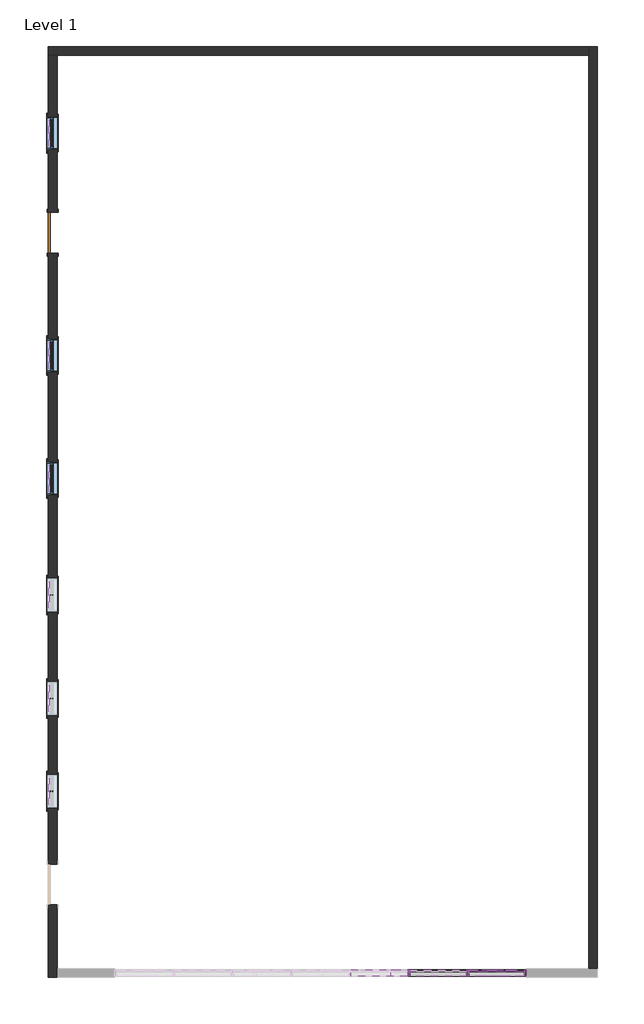
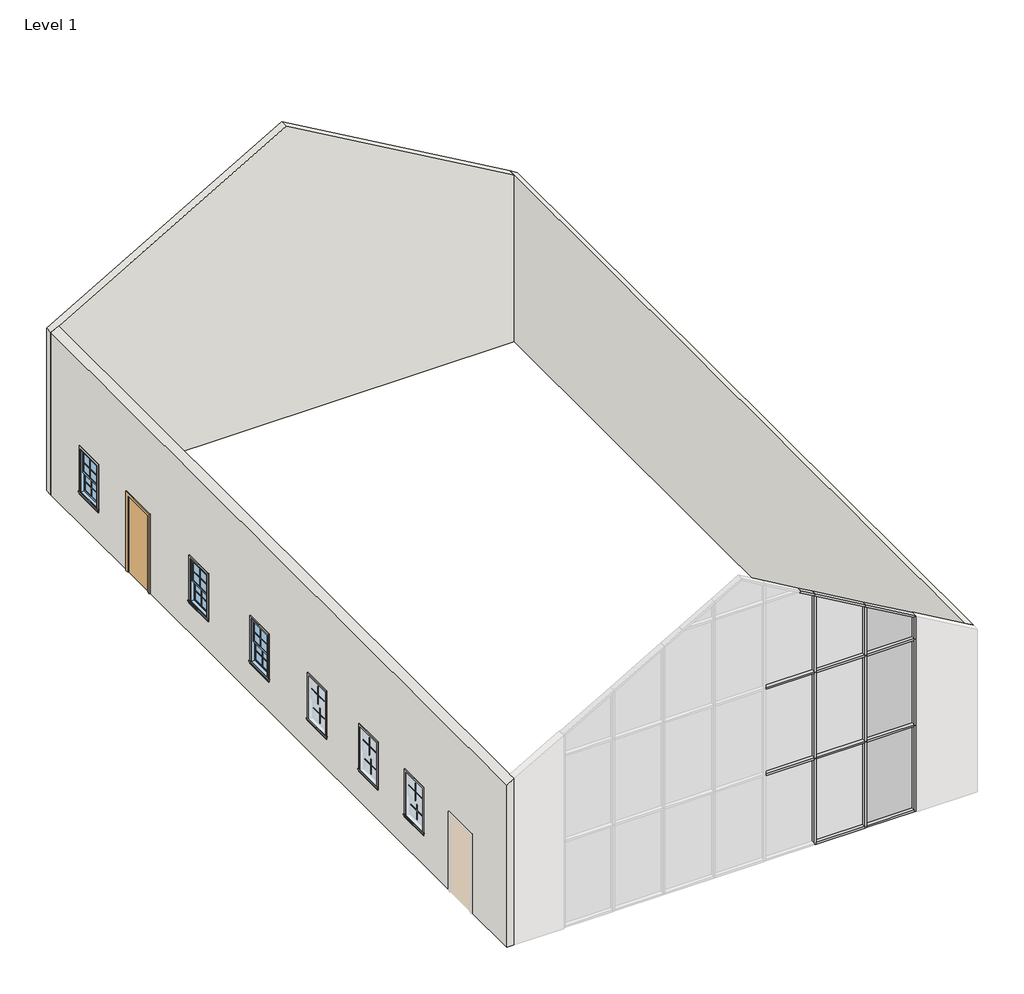
# One storey, part 2 of 2: 24 proxies, 20 members, 3 plates, 3 walls, 3 windows, 1 door.
"""IFC4 building model written with IfcOpenShell, lengths in millimetres."""

import ifcopenshell
import ifcopenshell.guid

model = None  # the IFC model being written
_history = None  # IfcOwnerHistory: only IFC2X3 demands one
_inside = {}  # id of a spatial element -> (the spatial element, [elements in it])
_under = {}  # id of a project, library or spatial element -> (it, [spatial elements below it])
_declared = {}  # id of a project -> (the project, [libraries it declares])
_typed = {}  # id of a type object -> (the type object, [elements of that type])
_made_of = {}  # id of a material, layer set ... -> (it, [elements and type objects made of it])


def new_model(schema):
    """Start an empty IFC model of exactly this schema.

    Asked for "IFC4X3", IfcOpenShell would pick the latest addendum, in which some entities
    have other attributes; the version numbers below select the first issue.
    IFC2X3 requires an IfcOwnerHistory on every rooted entity: one is made here for all.
    """
    global model, _history
    if schema == "IFC4X3":
        model = ifcopenshell.file(schema_version=(4, 3, 0, 0))
    else:
        model = ifcopenshell.file(schema=schema)
    _inside.clear()
    _under.clear()
    _declared.clear()
    _typed.clear()
    _made_of.clear()
    _history = None
    if model.schema == "IFC2X3":
        org = make("IfcOrganization", Name="unknown")
        user = make(
            "IfcPersonAndOrganization",
            ThePerson=make("IfcPerson", FamilyName="unknown"),
            TheOrganization=org,
        )
        app = make(
            "IfcApplication",
            ApplicationDeveloper=org,
            Version="unknown",
            ApplicationFullName="unknown",
            ApplicationIdentifier="unknown",
        )
        _history = make(
            "IfcOwnerHistory",
            OwningUser=user,
            OwningApplication=app,
            ChangeAction="ADDED",
            CreationDate=0,
        )
    return model


def make(cls, **values):
    """One entity of the class cls with the attributes given. An attribute that is None is left unset."""
    return model.create_entity(
        cls, **{name: value for name, value in values.items() if value is not None}
    )


def rooted(cls, **values):
    """An entity with a GlobalId (a new one), such as an element, a storey or a relation."""
    return make(cls, GlobalId=ifcopenshell.guid.new(), OwnerHistory=_history, **values)


def si_unit(unit_type, name, prefix=None):
    """IfcSIUnit, for example si_unit("LENGTHUNIT", "METRE", prefix="MILLI")."""
    return make("IfcSIUnit", UnitType=unit_type, Prefix=prefix, Name=name)


def assignment(units):
    """IfcUnitAssignment: the units of a project."""
    return None if units is None else make("IfcUnitAssignment", Units=units)


def point(xyz):
    """IfcCartesianPoint."""
    return None if xyz is None else make("IfcCartesianPoint", Coordinates=xyz)


def direction(xyz):
    """IfcDirection."""
    return None if xyz is None else make("IfcDirection", DirectionRatios=xyz)


def frame(location, z_axis=None, x_axis=None):
    """IfcAxis2Placement3D, a coordinate frame: its origin and axes. An axis left out is left unset."""
    return make(
        "IfcAxis2Placement3D",
        Location=point(location),
        Axis=direction(z_axis),
        RefDirection=direction(x_axis),
    )


def origin():
    """The frame at (0, 0, 0) with its axes left unset."""
    return frame((0.0, 0.0, 0.0))


def origin_with_axes():
    """The frame at (0, 0, 0) with the z axis (0, 0, 1) and the x axis (1, 0, 0) written out."""
    return frame((0.0, 0.0, 0.0), z_axis=(0.0, 0.0, 1.0), x_axis=(1.0, 0.0, 0.0))


def place(relative_to, where):
    """IfcLocalPlacement: puts the frame where relative to a parent placement (None: the world)."""
    return make(
        "IfcLocalPlacement", PlacementRelTo=relative_to, RelativePlacement=where
    )


def context(
    kind, dimensions, precision=None, world=None, true_north=None, identifier=None
):
    """IfcGeometricRepresentationContext, for example the 3D "Model" context."""
    return make(
        "IfcGeometricRepresentationContext",
        ContextIdentifier=identifier,
        ContextType=kind,
        CoordinateSpaceDimension=dimensions,
        Precision=precision,
        WorldCoordinateSystem=world,
        TrueNorth=true_north,
    )


def project(units=None, contexts=None):
    """IfcProject with its units and contexts."""
    return rooted(
        "IfcProject",
        Name="project",
        RepresentationContexts=contexts,
        UnitsInContext=assignment(units),
    )


def spatial(cls, under=None, at=None, **own):
    """A site, building, storey or space (cls), placed at a placement, below another one or the project."""
    s = rooted(cls, ObjectPlacement=at, **own)
    if under is not None:
        _under.setdefault(under.id(), (under, []))[1].append(s)
    return s


def polyline(points):
    """IfcPolyline through the points."""
    return make("IfcPolyline", Points=[point(p) for p in points])


def outline(outer, holes=None, kind="AREA"):
    """IfcArbitraryClosedProfileDef: a profile drawn as a closed curve; with holes, ...WithVoids."""
    if holes is None:
        return make("IfcArbitraryClosedProfileDef", ProfileType=kind, OuterCurve=outer)
    return make(
        "IfcArbitraryProfileDefWithVoids",
        ProfileType=kind,
        OuterCurve=outer,
        InnerCurves=holes,
    )


def extrude(swept, where, along, depth):
    """IfcExtrudedAreaSolid: the profile swept, set in the frame where, extruded along a direction by depth."""
    return make(
        "IfcExtrudedAreaSolid",
        SweptArea=swept,
        Position=where,
        ExtrudedDirection=direction(along),
        Depth=depth,
    )


def faces_of(points, faces, orient=None, outer=None):
    """IfcFace entities. A face is a list of loops; a loop is a list of indices into points, from 0.

    orient and outer hold one flag for each loop. By default every Orientation is true, the
    first loop of a face is its IfcFaceOuterBound and the others are IfcFaceBound.
    """
    made = []
    for i, loops in enumerate(faces):
        bounds = []
        for j, loop in enumerate(loops):
            is_outer = j == 0 if outer is None else outer[i][j]
            bounds.append(
                make(
                    "IfcFaceOuterBound" if is_outer else "IfcFaceBound",
                    Bound=make("IfcPolyLoop", Polygon=[points[k] for k in loop]),
                    Orientation=True if orient is None else orient[i][j],
                )
            )
        made.append(make("IfcFace", Bounds=bounds))
    return made


def faceted_brep(points, faces, orient=None, outer=None, voids=None):
    """IfcFacetedBrep: a solid bounded by flat faces; with voids (closed shells), ...WithVoids."""
    shared = [point(p) for p in points]
    hull = make("IfcClosedShell", CfsFaces=faces_of(shared, faces, orient, outer))
    if voids is None:
        return make("IfcFacetedBrep", Outer=hull)
    return make(
        "IfcFacetedBrepWithVoids",
        Outer=hull,
        Voids=[
            make(cls, CfsFaces=faces_of(shared, fs, o, b)) for cls, fs, o, b in voids
        ],
    )


def shape(context_of_items, identifier, shape_type, items):
    """IfcShapeRepresentation: the items that make up one representation, for example the "Body"."""
    return make(
        "IfcShapeRepresentation",
        ContextOfItems=context_of_items,
        RepresentationIdentifier=identifier,
        RepresentationType=shape_type,
        Items=items,
    )


def source(mapping_origin, context_of_items, identifier, shape_type, items):
    """IfcRepresentationMap: a shape defined once, which mapped items show again and again."""
    return make(
        "IfcRepresentationMap",
        MappingOrigin=mapping_origin,
        MappedRepresentation=shape(context_of_items, identifier, shape_type, items),
    )


def transform(
    local_origin,
    x_axis=None,
    y_axis=None,
    z_axis=None,
    scale=None,
    scale2=None,
    scale3=None,
    uniform=True,
):
    """IfcCartesianTransformationOperator3D, or its non-uniform kind. x_axis, y_axis, z_axis: its Axis1, 2, 3."""
    if uniform:
        return make(
            "IfcCartesianTransformationOperator3D",
            Axis1=direction(x_axis),
            Axis2=direction(y_axis),
            LocalOrigin=point(local_origin),
            Scale=scale,
            Axis3=direction(z_axis),
        )
    return make(
        "IfcCartesianTransformationOperator3DnonUniform",
        Axis1=direction(x_axis),
        Axis2=direction(y_axis),
        LocalOrigin=point(local_origin),
        Scale=scale,
        Axis3=direction(z_axis),
        Scale2=scale2,
        Scale3=scale3,
    )


def mapped(mapping_source, mapping_target):
    """IfcMappedItem: shows the shape of a source again, moved by a transform."""
    return make(
        "IfcMappedItem", MappingSource=mapping_source, MappingTarget=mapping_target
    )


def made_of(thing, what):
    """Note that an element or type object is made of a material, layer set ...; save() writes the relation."""
    if what is not None:
        _made_of.setdefault(what.id(), (what, []))[1].append(thing)
    return thing


def element(
    cls,
    number,
    at=None,
    inside=None,
    cuts=None,
    type_object=None,
    material=None,
    context=None,
    identifier="Body",
    shape_type=None,
    held_by="IfcProductDefinitionShape",
    body=None,
    shapes=None,
    **own,
):
    """One element of the class cls, such as IfcWall. Its Tag is "e" and its number.

    at: its placement. inside: the storey or other place that contains it. cuts: it is an
    opening in that element (IfcRelVoidsElement). A single representation is given by context,
    identifier, shape_type and body (its items); several are given by shapes. held_by: the class
    of the entity that holds the representations. save() writes the other relations.
    """
    e = rooted(cls, Tag="e%d" % number, ObjectPlacement=at, **own)
    if body is not None:
        shapes = [shape(context, identifier, shape_type, body)]
    if shapes is not None:
        e.Representation = make(held_by, Representations=shapes)
    if inside is not None:
        _inside.setdefault(inside.id(), (inside, []))[1].append(e)
    if cuts is not None:
        rooted(
            "IfcRelVoidsElement", RelatingBuildingElement=cuts, RelatedOpeningElement=e
        )
    if type_object is not None:
        _typed.setdefault(type_object.id(), (type_object, []))[1].append(e)
    return made_of(e, material)


def aggregate(whole, parts):
    """IfcRelAggregates: a whole, such as a stair, and the parts it consists of."""
    return rooted("IfcRelAggregates", RelatingObject=whole, RelatedObjects=parts)


def save(model, path):
    """Write the relations noted so far, then the file.

    IfcRelAggregates (storeys below a building ...), IfcRelContainedInSpatialStructure (elements
    in a storey), IfcRelDefinesByType, IfcRelAssociatesMaterial and IfcRelDeclares: one each for
    every whole, place, type object, material and project.
    """
    for whole, parts in _under.values():
        aggregate(whole, parts)
    for where, things in _inside.values():
        rooted(
            "IfcRelContainedInSpatialStructure",
            RelatedElements=things,
            RelatingStructure=where,
        )
    for kind, things in _typed.values():
        rooted("IfcRelDefinesByType", RelatedObjects=things, RelatingType=kind)
    for what, things in _made_of.values():
        rooted("IfcRelAssociatesMaterial", RelatedObjects=things, RelatingMaterial=what)
    for by, libraries in _declared.values():
        rooted("IfcRelDeclares", RelatingContext=by, RelatedDefinitions=libraries)
    model.write(path)


def m_muntin_pattern_2x2_m_muntin_pattern_2x2_aaec3afb(model_context):
    return source(origin(), model_context, "Body", "SweptSolid", [
        extrude(outline(polyline([(257.1375, -6.35), (257.1375, -298.8), (244.4375, -298.8), (244.4375, -6.35), (0.0, -6.35), (0.0, 6.35), (244.4375, 6.35), (244.4375, 298.8), (257.1375, 298.8), (257.1375, 6.35), (501.575, 6.35), (501.575, -6.35), (257.1375, -6.35)])), frame((0.0, 9.525, 0.0), z_axis=(0.0, 1.0, 0.0), x_axis=(0.0, 0.0, 1.0)), (0.0, 0.0, 1.0), 12.7),
        extrude(outline(polyline([(257.1375, -6.35), (257.1375, -298.8), (244.4375, -298.8), (244.4375, -6.35), (0.0, -6.35), (0.0, 6.35), (244.4375, 6.35), (244.4375, 298.8), (257.1375, 298.8), (257.1375, 6.35), (501.575, 6.35), (501.575, -6.35), (257.1375, -6.35)])), frame((0.0, -22.225, 0.0), z_axis=(0.0, 1.0, 0.0), x_axis=(0.0, 0.0, 1.0)), (0.0, 0.0, 1.0), 12.7),
    ])


def m_trim_window_exterior_flat_with_sill_e7ff6350(model_context):
    return source(origin(), model_context, "Body", "SweptSolid", [
        extrude(outline(polyline([(435.0, -1220.4323709), (435.0, -1280.4323709), (-435.0, -1280.4323709), (-435.0, -1220.4323709), (435.0, -1220.4323709)])), origin_with_axes(), (0.0, 0.0, 1.0), 19.05),
        extrude(outline(polyline([(-1230.0, 38.1), (-1202.4580645, 38.1), (-1200.0, 19.05), (-1200.0, 0.0), (-1220.4323709, 0.0), (-1220.4323709, 19.05), (-1230.0, 19.05), (-1230.0, 38.1)])), frame((-447.7, 0.0, 0.0), z_axis=(1.0, 0.0, 0.0), x_axis=(0.0, 1.0, 0.0)), (0.0, 0.0, 1.0), 895.4),
        extrude(outline(polyline([(-435.0, 60.0), (435.0, 60.0), (435.0, -1200.0), (375.0, -1200.0), (375.0, 0.0), (-375.0, 0.0), (-375.0, -1200.0), (-435.0, -1200.0), (-435.0, 60.0)])), origin_with_axes(), (0.0, 0.0, 1.0), 19.05),
    ])


def m_trim_window_interior_flat_picture_frame_31bd2320(model_context):
    return source(origin(), model_context, "Body", "SweptSolid", [
        extrude(outline(polyline([(422.3, 47.3), (422.3, -1247.3), (-422.3, -1247.3), (-422.3, 47.3), (422.3, 47.3)]), holes=[polyline([(362.3, -12.7), (-362.3, -12.7), (-362.3, -1187.3), (362.3, -1187.3), (362.3, -12.7)])]), origin_with_axes(), (0.0, 0.0, 1.0), 30.0),
    ])


def m_single_flush_0915_x_2134mm_6a9e8738(model_context):
    return source(origin(), model_context, "Body", "SweptSolid", [
        extrude(outline(polyline([(2210.0, -533.5), (0.0, -533.5), (0.0, -457.5), (2134.0, -457.5), (2134.0, 457.5), (0.0, 457.5), (0.0, 533.5), (2210.0, 533.5), (2210.0, -533.5)])), frame((0.0, 100.0, 0.0), z_axis=(0.0, 1.0, 0.0), x_axis=(0.0, 0.0, 1.0)), (0.0, 0.0, 1.0), 25.0),
        extrude(outline(polyline([(2210.0, 533.5), (2210.0, -533.5), (0.0, -533.5), (0.0, -457.5), (2134.0, -457.5), (2134.0, 457.5), (0.0, 457.5), (0.0, 533.5), (2210.0, 533.5)])), frame((0.0, -125.0, 0.0), z_axis=(0.0, 1.0, 0.0), x_axis=(0.0, 0.0, 1.0)), (0.0, 0.0, 1.0), 25.0),
        extrude(outline(polyline([(457.5, 49.0), (-457.5, 49.0), (-457.5, 100.0), (457.5, 100.0), (457.5, 49.0)])), origin_with_axes(), (0.0, 0.0, 1.0), 2134.0),
    ])


def rectangular_mullion_50mm_x_150mm_302a0cfa(model_context):
    return source(origin(), model_context, "Body", "SweptSolid", [
        extrude(outline(polyline([(0.0, 75.0), (0.0, -75.0), (-50.0, -75.0), (-50.0, 75.0), (0.0, 75.0)])), frame((0.0, 0.0, -1253.5714288), z_axis=(0.0, 0.0, 1.0), x_axis=(1.0, 0.0, 0.0)), (0.0, 0.0, 1.0), 1253.5714288),
    ])


def rectangular_mullion_50mm_x_150mm_11a5ee59(model_context):
    return source(origin(), model_context, "Body", "SweptSolid", [
        extrude(outline(polyline([(0.0, 75.0), (0.0, -75.0), (-50.0, -75.0), (-50.0, 75.0), (0.0, 75.0)])), frame((0.0, 0.0, -1278.5714285), z_axis=(0.0, 0.0, 1.0), x_axis=(1.0, 0.0, 0.0)), (0.0, 0.0, 1.0), 1278.5714285),
    ])


def rectangular_mullion_50mm_x_150mm_46426fc7(model_context):
    return source(origin(), model_context, "Body", "SweptSolid", [
        extrude(outline(polyline([(25.0, 75.0), (25.0, -75.0), (-25.0, -75.0), (-25.0, 75.0), (25.0, 75.0)])), frame((0.0, 0.0, -1253.5714288), z_axis=(0.0, 0.0, 1.0), x_axis=(1.0, 0.0, 0.0)), (0.0, 0.0, 1.0), 1253.5714288),
    ])


def rectangular_mullion_50mm_x_150mm_f38f42f6(model_context):
    return source(origin(), model_context, "Body", "SweptSolid", [
        extrude(outline(polyline([(25.0, 75.0), (25.0, -75.0), (-25.0, -75.0), (-25.0, 75.0), (25.0, 75.0)])), frame((0.0, 0.0, -1278.5714285), z_axis=(0.0, 0.0, 1.0), x_axis=(1.0, 0.0, 0.0)), (0.0, 0.0, 1.0), 1278.5714285),
    ])


def rectangular_mullion_50mm_x_150mm_6225e4e3(model_context):
    return source(origin(), model_context, "Body", "SweptSolid", [
        extrude(outline(polyline([(25.0, 75.0), (25.0, -75.0), (-25.0, -75.0), (-25.0, 75.0), (25.0, 75.0)])), frame((0.0, 0.0, -2400.0), z_axis=(0.0, 0.0, 1.0), x_axis=(1.0, 0.0, 0.0)), (0.0, 0.0, 1.0), 2400.0),
    ])


def rectangular_mullion_50mm_x_150mm_662c37b1(model_context):
    return source(origin(), model_context, "Body", "SweptSolid", [
        extrude(outline(polyline([(0.0, 75.0), (0.0, -75.0), (-50.0, -75.0), (-50.0, 75.0), (0.0, 75.0)])), frame((0.0, 0.0, -2400.0), z_axis=(0.0, 0.0, 1.0), x_axis=(1.0, 0.0, 0.0)), (0.0, 0.0, 1.0), 2400.0),
    ])


def rectangular_mullion_50mm_x_150mm_c4d7f9a4(model_context):
    return source(origin(), model_context, "Body", "SweptSolid", [
        extrude(outline(polyline([(0.0, 25.0), (0.0, -25.0), (-2134.1765467, -25.0), (-2105.3090332, 25.0), (0.0, 25.0)])), frame((0.0, -75.0, 0.0), z_axis=(0.0, 1.0, 0.0), x_axis=(0.0, 0.0, 1.0)), (0.0, 0.0, 1.0), 150.0),
    ])


def rectangular_mullion_50mm_x_150mm_5374cabd(model_context):
    return source(origin(), model_context, "Body", "SweptSolid", [
        extrude(outline(polyline([(0.0, 25.0), (0.0, -25.0), (-1367.1254748, -25.0), (-1338.2579614, 25.0), (0.0, 25.0)])), frame((0.0, -75.0, 0.0), z_axis=(0.0, 1.0, 0.0), x_axis=(0.0, 0.0, 1.0)), (0.0, 0.0, 1.0), 150.0),
    ])


def rectangular_mullion_50mm_x_150mm_03c50f69(model_context):
    return source(origin(), model_context, "Body", "SweptSolid", [
        extrude(outline(polyline([(0.0, 0.0), (-28.8675135, -50.0), (-1534.1021441, -50.0), (-1534.1021441, 0.0), (0.0, 0.0)])), frame((0.0, -75.0, 0.0), z_axis=(0.0, 1.0, 0.0), x_axis=(0.0, 0.0, 1.0)), (0.0, 0.0, 1.0), 150.0),
    ])


def rectangular_mullion_50mm_x_150mm_ffb0b627(model_context):
    return source(origin(), model_context, "Body", "SweptSolid", [
        extrude(outline(polyline([(0.0, 75.0), (0.0, -75.0), (-50.0, -75.0), (-50.0, 75.0), (0.0, 75.0)])), frame((0.0, 0.0, -445.0443662), z_axis=(0.0, 0.0, 1.0), x_axis=(1.0, 0.0, 0.0)), (0.0, 0.0, 1.0), 445.0443662),
    ])


def rectangular_mullion_50mm_x_150mm_95afd124(model_context):
    return source(origin(), model_context, "Body", "SweptSolid", [
        extrude(outline(polyline([(0.0, 75.0), (0.0, -75.0), (-50.0, -75.0), (-50.0, 75.0), (0.0, 75.0)])), frame((0.0, 0.0, -1534.1021437), z_axis=(0.0, 0.0, 1.0), x_axis=(1.0, 0.0, 0.0)), (0.0, 0.0, 1.0), 1534.1021437),
    ])


def rectangular_mullion_50mm_x_150mm_b704ab83(model_context):
    return source(origin(), model_context, "Body", "SweptSolid", [
        extrude(outline(polyline([(0.0, 0.0), (0.0, -50.0), (-614.5081595, -50.0), (-643.375673, 0.0), (0.0, 0.0)])), frame((0.0, -75.0, 0.0), z_axis=(0.0, 1.0, 0.0), x_axis=(0.0, 0.0, 1.0)), (0.0, 0.0, 1.0), 150.0),
    ])


def system_panel_glazed_b60b372a(model_context):
    return source(origin(), model_context, "Body", "SweptSolid", [
        extrude(outline(polyline([(626.7857144, 24.5), (-626.7857144, 24.5), (-626.7857144, 49.5), (626.7857144, 49.5), (626.7857144, 24.5)])), origin_with_axes(), (0.0, 0.0, 1.0), 2325.0),
    ])


def system_panel_glazed_eec4e8b3(model_context):
    return source(origin(), model_context, "Body", "SweptSolid", [
        extrude(outline(polyline([(626.7857144, 24.5), (-626.7857144, 24.5), (-626.7857144, 49.5), (626.7857144, 49.5), (626.7857144, 24.5)])), origin_with_axes(), (0.0, 0.0, 1.0), 2350.0),
    ])


def system_panel_glazed_62c7097b(model_context):
    return source(origin(), model_context, "Body", "SweptSolid", [
        extrude(outline(polyline([(0.0, -626.7857144), (0.0, 626.7857144), (589.5081595, 626.7857144), (1313.2579614, -626.7857144), (0.0, -626.7857144)])), frame((0.0, 24.5, 0.0), z_axis=(0.0, 1.0, 0.0), x_axis=(0.0, 0.0, 1.0)), (0.0, 0.0, 1.0), 25.0),
    ])


def m_window_double_hung_750_x_1200mm_41070976(model_context):
    return source(origin(), model_context, "Body", "SweptSolid", [
        extrude(outline(polyline([(298.8, 30.15), (298.8, 23.8), (-298.8, 23.8), (-298.8, 30.15), (298.8, 30.15)])), frame((0.0, 0.0, 990.6), z_axis=(0.0, 0.0, 1.0), x_axis=(1.0, 0.0, 0.0)), (0.0, 0.0, 1.0), 501.575),
        extrude(outline(polyline([(-298.8, 17.45), (298.8, 17.45), (298.8, 11.1), (-298.8, 11.1), (-298.8, 17.45)])), frame((0.0, 0.0, 990.6), z_axis=(0.0, 0.0, 1.0), x_axis=(1.0, 0.0, 0.0)), (0.0, 0.0, 1.0), 501.575),
        extrude(outline(polyline([(298.8, 74.6), (298.8, 68.25), (-298.8, 68.25), (-298.8, 74.6), (298.8, 74.6)])), frame((0.0, 0.0, 1536.625), z_axis=(0.0, 0.0, 1.0), x_axis=(1.0, 0.0, 0.0)), (0.0, 0.0, 1.0), 501.575),
        extrude(outline(polyline([(-298.8, 61.9), (298.8, 61.9), (298.8, 55.55), (-298.8, 55.55), (-298.8, 61.9)])), frame((0.0, 0.0, 1536.625), z_axis=(0.0, 0.0, 1.0), x_axis=(1.0, 0.0, 0.0)), (0.0, 0.0, 1.0), 501.575),
        extrude(outline(polyline([(1536.625, -343.25), (946.15, -343.25), (946.15, 343.25), (1536.625, 343.25), (1536.625, -343.25)]), holes=[polyline([(1492.175, 298.8), (990.6, 298.8), (990.6, -298.8), (1492.175, -298.8), (1492.175, 298.8)])]), frame((0.0, -1.6, 0.0), z_axis=(0.0, 1.0, 0.0), x_axis=(0.0, 0.0, 1.0)), (0.0, 0.0, 1.0), 44.45),
        extrude(outline(polyline([(2082.65, -343.25), (1492.175, -343.25), (1492.175, 343.25), (2082.65, 343.25), (2082.65, -343.25)]), holes=[polyline([(2038.2, 298.8), (1536.625, 298.8), (1536.625, -298.8), (2038.2, -298.8), (2038.2, 298.8)])]), frame((0.0, 42.85, 0.0), z_axis=(0.0, 1.0, 0.0), x_axis=(0.0, 0.0, 1.0)), (0.0, 0.0, 1.0), 44.45),
        extrude(outline(polyline([(2114.4, -375.0), (914.4, -375.0), (914.4, 375.0), (2114.4, 375.0), (2114.4, -375.0)]), holes=[polyline([(2082.65, 343.25), (946.15, 343.25), (946.15, -343.25), (2082.65, -343.25), (2082.65, 343.25)])]), frame((0.0, -14.3, 0.0), z_axis=(0.0, 1.0, 0.0), x_axis=(0.0, 0.0, 1.0)), (0.0, 0.0, 1.0), 133.35),
        extrude(outline(polyline([(2114.4, 375.0), (2114.4, -375.0), (914.4, -375.0), (914.4, 375.0), (2114.4, 375.0)]), holes=[polyline([(2095.35, 355.95), (933.45, 355.95), (933.45, -355.95), (2095.35, -355.95), (2095.35, 355.95)])]), frame((0.0, -100.0, 0.0), z_axis=(0.0, 1.0, 0.0), x_axis=(0.0, 0.0, 1.0)), (0.0, 0.0, 1.0), 85.7),
    ])


model = new_model("IFC4")

# Units and contexts
model_context = context("Model", 3, world=origin())
ifc_project = project(units=[si_unit("LENGTHUNIT", "METRE", prefix="MILLI")], contexts=[model_context])

# Site, building, storey
site = spatial("IfcSite", under=ifc_project)
building = spatial("IfcBuilding", under=site)
storey = spatial("IfcBuildingStorey", under=building, Name="Level 1", Elevation=0.0)

# Proxies
placement = place(None, origin())
m_muntin_pattern_2x2_m_muntin_pattern_2x2_shape = m_muntin_pattern_2x2_m_muntin_pattern_2x2_aaec3afb(model_context)
element("IfcBuildingElementProxy", 1, Name="M_Muntin Pattern_2x2 : M_Muntin Pattern_2x2", ObjectType="M_Muntin Pattern_2x2 : M_Muntin Pattern_2x2", at=placement, inside=storey, context=model_context, shape_type="MappedRepresentation", body=[
    mapped(m_muntin_pattern_2x2_m_muntin_pattern_2x2_shape, transform((-7032.909392, -4566.9793434, 1536.625), x_axis=(0.0, 1.0, 0.0), y_axis=(-1.0, 0.0, 0.0), z_axis=(0.0, 0.0, 1.0))),
])
element("IfcBuildingElementProxy", 2, Name="M_Muntin Pattern_2x2 : M_Muntin Pattern_2x2", ObjectType="M_Muntin Pattern_2x2 : M_Muntin Pattern_2x2", at=placement, inside=storey, context=model_context, shape_type="MappedRepresentation", body=[
    mapped(m_muntin_pattern_2x2_m_muntin_pattern_2x2_shape, transform((-6988.459392, -4566.9793434, 990.6), x_axis=(0.0, 1.0, 0.0), y_axis=(-1.0, 0.0, 0.0), z_axis=(0.0, 0.0, 1.0))),
])
element("IfcBuildingElementProxy", 3, Name="M_Muntin Pattern_2x2 : M_Muntin Pattern_2x2", ObjectType="M_Muntin Pattern_2x2 : M_Muntin Pattern_2x2", at=placement, inside=storey, context=model_context, shape_type="MappedRepresentation", body=[
    mapped(m_muntin_pattern_2x2_m_muntin_pattern_2x2_shape, transform((-7032.909392, -2474.0000934, 1536.625), x_axis=(0.0, 1.0, 0.0), y_axis=(-1.0, 0.0, 0.0), z_axis=(0.0, 0.0, 1.0))),
])
element("IfcBuildingElementProxy", 4, Name="M_Muntin Pattern_2x2 : M_Muntin Pattern_2x2", ObjectType="M_Muntin Pattern_2x2 : M_Muntin Pattern_2x2", at=placement, inside=storey, context=model_context, shape_type="MappedRepresentation", body=[
    mapped(m_muntin_pattern_2x2_m_muntin_pattern_2x2_shape, transform((-6988.459392, -2474.0000934, 990.6), x_axis=(0.0, 1.0, 0.0), y_axis=(-1.0, 0.0, 0.0), z_axis=(0.0, 0.0, 1.0))),
])
element("IfcBuildingElementProxy", 5, Name="M_Muntin Pattern_2x2 : M_Muntin Pattern_2x2", ObjectType="M_Muntin Pattern_2x2 : M_Muntin Pattern_2x2", at=placement, inside=storey, context=model_context, shape_type="MappedRepresentation", body=[
    mapped(m_muntin_pattern_2x2_m_muntin_pattern_2x2_shape, transform((-7032.909392, -137.6511631, 1536.625), x_axis=(0.0, 1.0, 0.0), y_axis=(-1.0, 0.0, 0.0), z_axis=(0.0, 0.0, 1.0))),
])
element("IfcBuildingElementProxy", 6, Name="M_Muntin Pattern_2x2 : M_Muntin Pattern_2x2", ObjectType="M_Muntin Pattern_2x2 : M_Muntin Pattern_2x2", at=placement, inside=storey, context=model_context, shape_type="MappedRepresentation", body=[
    mapped(m_muntin_pattern_2x2_m_muntin_pattern_2x2_shape, transform((-6988.459392, -137.6511631, 990.6), x_axis=(0.0, 1.0, 0.0), y_axis=(-1.0, 0.0, 0.0), z_axis=(0.0, 0.0, 1.0))),
])
element("IfcBuildingElementProxy", 7, Name="M_Muntin Pattern_2x2 : M_Muntin Pattern_2x2", ObjectType="M_Muntin Pattern_2x2 : M_Muntin Pattern_2x2", at=placement, inside=storey, context=model_context, shape_type="MappedRepresentation", body=[
    mapped(m_muntin_pattern_2x2_m_muntin_pattern_2x2_shape, transform((-7032.909392, 2490.7413834, 1536.625), x_axis=(0.0, 1.0, 0.0), y_axis=(-1.0, 0.0, 0.0), z_axis=(0.0, 0.0, 1.0))),
])
element("IfcBuildingElementProxy", 8, Name="M_Muntin Pattern_2x2 : M_Muntin Pattern_2x2", ObjectType="M_Muntin Pattern_2x2 : M_Muntin Pattern_2x2", at=placement, inside=storey, context=model_context, shape_type="MappedRepresentation", body=[
    mapped(m_muntin_pattern_2x2_m_muntin_pattern_2x2_shape, transform((-6988.459392, 2490.7413834, 990.6), x_axis=(0.0, 1.0, 0.0), y_axis=(-1.0, 0.0, 0.0), z_axis=(0.0, 0.0, 1.0))),
])
element("IfcBuildingElementProxy", 9, Name="M_Muntin Pattern_2x2 : M_Muntin Pattern_2x2", ObjectType="M_Muntin Pattern_2x2 : M_Muntin Pattern_2x2", at=placement, inside=storey, context=model_context, shape_type="MappedRepresentation", body=[
    mapped(m_muntin_pattern_2x2_m_muntin_pattern_2x2_shape, transform((-7032.909392, 5265.1557382, 1536.625), x_axis=(0.0, 1.0, 0.0), y_axis=(-1.0, 0.0, 0.0), z_axis=(0.0, 0.0, 1.0))),
])
element("IfcBuildingElementProxy", 10, Name="M_Muntin Pattern_2x2 : M_Muntin Pattern_2x2", ObjectType="M_Muntin Pattern_2x2 : M_Muntin Pattern_2x2", at=placement, inside=storey, context=model_context, shape_type="MappedRepresentation", body=[
    mapped(m_muntin_pattern_2x2_m_muntin_pattern_2x2_shape, transform((-6988.459392, 5265.1557382, 990.6), x_axis=(0.0, 1.0, 0.0), y_axis=(-1.0, 0.0, 0.0), z_axis=(0.0, 0.0, 1.0))),
])
element("IfcBuildingElementProxy", 11, Name="M_Muntin Pattern_2x2 : M_Muntin Pattern_2x2", ObjectType="M_Muntin Pattern_2x2 : M_Muntin Pattern_2x2", at=placement, inside=storey, context=model_context, shape_type="MappedRepresentation", body=[
    mapped(m_muntin_pattern_2x2_m_muntin_pattern_2x2_shape, transform((-7032.909392, 10278.571151, 1536.625), x_axis=(0.0, 1.0, 0.0), y_axis=(-1.0, 0.0, 0.0), z_axis=(0.0, 0.0, 1.0))),
])
element("IfcBuildingElementProxy", 12, Name="M_Muntin Pattern_2x2 : M_Muntin Pattern_2x2", ObjectType="M_Muntin Pattern_2x2 : M_Muntin Pattern_2x2", at=placement, inside=storey, context=model_context, shape_type="MappedRepresentation", body=[
    mapped(m_muntin_pattern_2x2_m_muntin_pattern_2x2_shape, transform((-6988.459392, 10278.571151, 990.6), x_axis=(0.0, 1.0, 0.0), y_axis=(-1.0, 0.0, 0.0), z_axis=(0.0, 0.0, 1.0))),
])
m_trim_window_exterior_flat_with_sill_shape = m_trim_window_exterior_flat_with_sill_e7ff6350(model_context)
element("IfcBuildingElementProxy", 13, Name="M_Trim-Window-Exterior-Flat : with Sill", ObjectType="M_Trim-Window-Exterior-Flat : with Sill", at=placement, inside=storey, context=model_context, shape_type="MappedRepresentation", body=[
    mapped(m_trim_window_exterior_flat_with_sill_shape, transform((-7067.834392, -4566.9793434, 2114.4), x_axis=(0.0, -1.0, 0.0), y_axis=(0.0, 0.0, 1.0), z_axis=(-1.0, 0.0, 0.0))),
])
element("IfcBuildingElementProxy", 14, Name="M_Trim-Window-Exterior-Flat : with Sill", ObjectType="M_Trim-Window-Exterior-Flat : with Sill", at=placement, inside=storey, context=model_context, shape_type="MappedRepresentation", body=[
    mapped(m_trim_window_exterior_flat_with_sill_shape, transform((-7067.834392, -2474.0000934, 2114.4), x_axis=(0.0, -1.0, 0.0), y_axis=(0.0, 0.0, 1.0), z_axis=(-1.0, 0.0, 0.0))),
])
element("IfcBuildingElementProxy", 15, Name="M_Trim-Window-Exterior-Flat : with Sill", ObjectType="M_Trim-Window-Exterior-Flat : with Sill", at=placement, inside=storey, context=model_context, shape_type="MappedRepresentation", body=[
    mapped(m_trim_window_exterior_flat_with_sill_shape, transform((-7067.834392, -137.6511631, 2114.4), x_axis=(0.0, -1.0, 0.0), y_axis=(0.0, 0.0, 1.0), z_axis=(-1.0, 0.0, 0.0))),
])
element("IfcBuildingElementProxy", 16, Name="M_Trim-Window-Exterior-Flat : with Sill", ObjectType="M_Trim-Window-Exterior-Flat : with Sill", at=placement, inside=storey, context=model_context, shape_type="MappedRepresentation", body=[
    mapped(m_trim_window_exterior_flat_with_sill_shape, transform((-7067.834392, 2490.7413834, 2114.4), x_axis=(0.0, -1.0, 0.0), y_axis=(0.0, 0.0, 1.0), z_axis=(-1.0, 0.0, 0.0))),
])
element("IfcBuildingElementProxy", 17, Name="M_Trim-Window-Exterior-Flat : with Sill", ObjectType="M_Trim-Window-Exterior-Flat : with Sill", at=placement, inside=storey, context=model_context, shape_type="MappedRepresentation", body=[
    mapped(m_trim_window_exterior_flat_with_sill_shape, transform((-7067.834392, 5265.1557382, 2114.4), x_axis=(0.0, -1.0, 0.0), y_axis=(0.0, 0.0, 1.0), z_axis=(-1.0, 0.0, 0.0))),
])
element("IfcBuildingElementProxy", 18, Name="M_Trim-Window-Exterior-Flat : with Sill", ObjectType="M_Trim-Window-Exterior-Flat : with Sill", at=placement, inside=storey, context=model_context, shape_type="MappedRepresentation", body=[
    mapped(m_trim_window_exterior_flat_with_sill_shape, transform((-7067.834392, 10278.571151, 2114.4), x_axis=(0.0, -1.0, 0.0), y_axis=(0.0, 0.0, 1.0), z_axis=(-1.0, 0.0, 0.0))),
])
m_trim_window_interior_flat_picture_frame_shape = m_trim_window_interior_flat_picture_frame_31bd2320(model_context)
element("IfcBuildingElementProxy", 19, Name="M_Trim-Window-Interior-Flat : Picture Frame", ObjectType="M_Trim-Window-Interior-Flat : Picture Frame", at=placement, inside=storey, context=model_context, shape_type="MappedRepresentation", body=[
    mapped(m_trim_window_interior_flat_picture_frame_shape, transform((-6867.834392, -4566.9793434, 2114.4), x_axis=(0.0, 1.0, 0.0), y_axis=(0.0, 0.0, 1.0), z_axis=(1.0, 0.0, 0.0))),
])
element("IfcBuildingElementProxy", 20, Name="M_Trim-Window-Interior-Flat : Picture Frame", ObjectType="M_Trim-Window-Interior-Flat : Picture Frame", at=placement, inside=storey, context=model_context, shape_type="MappedRepresentation", body=[
    mapped(m_trim_window_interior_flat_picture_frame_shape, transform((-6867.834392, -2474.0000934, 2114.4), x_axis=(0.0, 1.0, 0.0), y_axis=(0.0, 0.0, 1.0), z_axis=(1.0, 0.0, 0.0))),
])
element("IfcBuildingElementProxy", 21, Name="M_Trim-Window-Interior-Flat : Picture Frame", ObjectType="M_Trim-Window-Interior-Flat : Picture Frame", at=placement, inside=storey, context=model_context, shape_type="MappedRepresentation", body=[
    mapped(m_trim_window_interior_flat_picture_frame_shape, transform((-6867.834392, -137.6511631, 2114.4), x_axis=(0.0, 1.0, 0.0), y_axis=(0.0, 0.0, 1.0), z_axis=(1.0, 0.0, 0.0))),
])
element("IfcBuildingElementProxy", 22, Name="M_Trim-Window-Interior-Flat : Picture Frame", ObjectType="M_Trim-Window-Interior-Flat : Picture Frame", at=placement, inside=storey, context=model_context, shape_type="MappedRepresentation", body=[
    mapped(m_trim_window_interior_flat_picture_frame_shape, transform((-6867.834392, 2490.7413834, 2114.4), x_axis=(0.0, 1.0, 0.0), y_axis=(0.0, 0.0, 1.0), z_axis=(1.0, 0.0, 0.0))),
])
element("IfcBuildingElementProxy", 23, Name="M_Trim-Window-Interior-Flat : Picture Frame", ObjectType="M_Trim-Window-Interior-Flat : Picture Frame", at=placement, inside=storey, context=model_context, shape_type="MappedRepresentation", body=[
    mapped(m_trim_window_interior_flat_picture_frame_shape, transform((-6867.834392, 5265.1557382, 2114.4), x_axis=(0.0, 1.0, 0.0), y_axis=(0.0, 0.0, 1.0), z_axis=(1.0, 0.0, 0.0))),
])
element("IfcBuildingElementProxy", 24, Name="M_Trim-Window-Interior-Flat : Picture Frame", ObjectType="M_Trim-Window-Interior-Flat : Picture Frame", at=placement, inside=storey, context=model_context, shape_type="MappedRepresentation", body=[
    mapped(m_trim_window_interior_flat_picture_frame_shape, transform((-6867.834392, 10278.571151, 2114.4), x_axis=(0.0, 1.0, 0.0), y_axis=(0.0, 0.0, 1.0), z_axis=(1.0, 0.0, 0.0))),
])

# Door
m_single_flush_0915_x_2134mm_shape = m_single_flush_0915_x_2134mm_6a9e8738(model_context)
element("IfcDoor", 25, ObjectType="M_Single-Flush : 0915 x 2134mm", at=placement, inside=storey, context=model_context, shape_type="MappedRepresentation", body=[
    mapped(m_single_flush_0915_x_2134mm_shape, transform((-6967.834392, 8033.0206566, 0.0), x_axis=(0.0, 1.0, 0.0), y_axis=(-1.0, 0.0, 0.0), z_axis=(0.0, 0.0, 1.0))),
])

# Members
rectangular_mullion_50mm_x_150mm_shape = rectangular_mullion_50mm_x_150mm_302a0cfa(model_context)
element("IfcMember", 26, ObjectType="Rectangular Mullion : 50mm x 150mm", at=placement, inside=storey, context=model_context, shape_type="MappedRepresentation", body=[
    mapped(rectangular_mullion_50mm_x_150mm_shape, transform((2428.5941792, -8666.9793434, 0.0), x_axis=(0.0, 0.0, -1.0), y_axis=(0.0, -1.0, 0.0), z_axis=(-1.0, 0.0, 0.0))),
])
rectangular_mullion_50mm_x_150mm_2_shape = rectangular_mullion_50mm_x_150mm_11a5ee59(model_context)
element("IfcMember", 27, ObjectType="Rectangular Mullion : 50mm x 150mm", at=placement, inside=storey, context=model_context, shape_type="MappedRepresentation", body=[
    mapped(rectangular_mullion_50mm_x_150mm_2_shape, transform((1100.0227508, -8666.9793434, 0.0), x_axis=(0.0, 0.0, -1.0), y_axis=(0.0, -1.0, 0.0), z_axis=(-1.0, 0.0, 0.0))),
])
rectangular_mullion_50mm_x_150mm_3_shape = rectangular_mullion_50mm_x_150mm_46426fc7(model_context)
element("IfcMember", 28, ObjectType="Rectangular Mullion : 50mm x 150mm", at=placement, inside=storey, context=model_context, shape_type="MappedRepresentation", body=[
    mapped(rectangular_mullion_50mm_x_150mm_3_shape, transform((3682.165608, -8666.9793434, 2400.0), x_axis=(0.0, 0.0, 1.0), y_axis=(0.0, -1.0, 0.0), z_axis=(1.0, 0.0, 0.0))),
])
element("IfcMember", 29, ObjectType="Rectangular Mullion : 50mm x 150mm", at=placement, inside=storey, context=model_context, shape_type="MappedRepresentation", body=[
    mapped(rectangular_mullion_50mm_x_150mm_3_shape, transform((3682.165608, -8666.9793434, 4800.0), x_axis=(0.0, 0.0, 1.0), y_axis=(0.0, -1.0, 0.0), z_axis=(1.0, 0.0, 0.0))),
])
rectangular_mullion_50mm_x_150mm_4_shape = rectangular_mullion_50mm_x_150mm_f38f42f6(model_context)
element("IfcMember", 30, ObjectType="Rectangular Mullion : 50mm x 150mm", at=placement, inside=storey, context=model_context, shape_type="MappedRepresentation", body=[
    mapped(rectangular_mullion_50mm_x_150mm_4_shape, transform((1050.0227508, -8666.9793434, 2400.0), x_axis=(0.0, 0.0, 1.0), y_axis=(0.0, -1.0, 0.0), z_axis=(1.0, 0.0, 0.0))),
])
element("IfcMember", 31, ObjectType="Rectangular Mullion : 50mm x 150mm", at=placement, inside=storey, context=model_context, shape_type="MappedRepresentation", body=[
    mapped(rectangular_mullion_50mm_x_150mm_4_shape, transform((2378.5941792, -8666.9793434, 2400.0), x_axis=(0.0, 0.0, 1.0), y_axis=(0.0, -1.0, 0.0), z_axis=(1.0, 0.0, 0.0))),
])
element("IfcMember", 32, ObjectType="Rectangular Mullion : 50mm x 150mm", at=placement, inside=storey, context=model_context, shape_type="MappedRepresentation", body=[
    mapped(rectangular_mullion_50mm_x_150mm_4_shape, transform((1050.0227508, -8666.9793434, 4800.0), x_axis=(0.0, 0.0, 1.0), y_axis=(0.0, -1.0, 0.0), z_axis=(1.0, 0.0, 0.0))),
])
element("IfcMember", 33, ObjectType="Rectangular Mullion : 50mm x 150mm", at=placement, inside=storey, context=model_context, shape_type="MappedRepresentation", body=[
    mapped(rectangular_mullion_50mm_x_150mm_4_shape, transform((2378.5941792, -8666.9793434, 4800.0), x_axis=(0.0, 0.0, 1.0), y_axis=(0.0, -1.0, 0.0), z_axis=(1.0, 0.0, 0.0))),
])
rectangular_mullion_50mm_x_150mm_5_shape = rectangular_mullion_50mm_x_150mm_6225e4e3(model_context)
element("IfcMember", 34, ObjectType="Rectangular Mullion : 50mm x 150mm", at=placement, inside=storey, context=model_context, shape_type="MappedRepresentation", body=[
    mapped(rectangular_mullion_50mm_x_150mm_5_shape, transform((1075.0227508, -8666.9793434, 0.0), x_axis=(1.0, 0.0, 0.0), y_axis=(0.0, -1.0, 0.0), z_axis=(0.0, 0.0, -1.0))),
])
element("IfcMember", 35, ObjectType="Rectangular Mullion : 50mm x 150mm", at=placement, inside=storey, context=model_context, shape_type="MappedRepresentation", body=[
    mapped(rectangular_mullion_50mm_x_150mm_5_shape, transform((2403.5941792, -8666.9793434, 0.0), x_axis=(1.0, 0.0, 0.0), y_axis=(0.0, -1.0, 0.0), z_axis=(0.0, 0.0, -1.0))),
])
element("IfcMember", 36, ObjectType="Rectangular Mullion : 50mm x 150mm", at=placement, inside=storey, context=model_context, shape_type="MappedRepresentation", body=[
    mapped(rectangular_mullion_50mm_x_150mm_5_shape, transform((1075.0227508, -8666.9793434, 2400.0), x_axis=(1.0, 0.0, 0.0), y_axis=(0.0, -1.0, 0.0), z_axis=(0.0, 0.0, -1.0))),
])
element("IfcMember", 37, ObjectType="Rectangular Mullion : 50mm x 150mm", at=placement, inside=storey, context=model_context, shape_type="MappedRepresentation", body=[
    mapped(rectangular_mullion_50mm_x_150mm_5_shape, transform((2403.5941792, -8666.9793434, 2400.0), x_axis=(1.0, 0.0, 0.0), y_axis=(0.0, -1.0, 0.0), z_axis=(0.0, 0.0, -1.0))),
])
rectangular_mullion_50mm_x_150mm_6_shape = rectangular_mullion_50mm_x_150mm_662c37b1(model_context)
element("IfcMember", 38, ObjectType="Rectangular Mullion : 50mm x 150mm", at=placement, inside=storey, context=model_context, shape_type="MappedRepresentation", body=[
    mapped(rectangular_mullion_50mm_x_150mm_6_shape, transform((3732.165608, -8666.9793434, 0.0), x_axis=(1.0, 0.0, 0.0), y_axis=(0.0, -1.0, 0.0), z_axis=(0.0, 0.0, -1.0))),
])
element("IfcMember", 39, ObjectType="Rectangular Mullion : 50mm x 150mm", at=placement, inside=storey, context=model_context, shape_type="MappedRepresentation", body=[
    mapped(rectangular_mullion_50mm_x_150mm_6_shape, transform((3732.165608, -8666.9793434, 2400.0), x_axis=(1.0, 0.0, 0.0), y_axis=(0.0, -1.0, 0.0), z_axis=(0.0, 0.0, -1.0))),
])
rectangular_mullion_50mm_x_150mm_7_shape = rectangular_mullion_50mm_x_150mm_c4d7f9a4(model_context)
element("IfcMember", 40, ObjectType="Rectangular Mullion : 50mm x 150mm", at=placement, inside=storey, context=model_context, shape_type="MappedRepresentation", body=[
    mapped(rectangular_mullion_50mm_x_150mm_7_shape, transform((1075.0227508, -8666.9793434, 4800.0), x_axis=(1.0, 0.0, 0.0), y_axis=(0.0, -1.0, 0.0), z_axis=(0.0, 0.0, -1.0))),
])
rectangular_mullion_50mm_x_150mm_8_shape = rectangular_mullion_50mm_x_150mm_5374cabd(model_context)
element("IfcMember", 41, ObjectType="Rectangular Mullion : 50mm x 150mm", at=placement, inside=storey, context=model_context, shape_type="MappedRepresentation", body=[
    mapped(rectangular_mullion_50mm_x_150mm_8_shape, transform((2403.5941792, -8666.9793434, 4800.0), x_axis=(1.0, 0.0, 0.0), y_axis=(0.0, -1.0, 0.0), z_axis=(0.0, 0.0, -1.0))),
])
rectangular_mullion_50mm_x_150mm_9_shape = rectangular_mullion_50mm_x_150mm_03c50f69(model_context)
element("IfcMember", 42, ObjectType="Rectangular Mullion : 50mm x 150mm", at=placement, inside=storey, context=model_context, shape_type="MappedRepresentation", body=[
    mapped(rectangular_mullion_50mm_x_150mm_9_shape, transform((3732.165608, -8666.9793434, 5443.375673), x_axis=(0.5000000000000007, 0.0, 0.8660254037844384), y_axis=(0.0, -1.0, 0.0), z_axis=(0.8660254037844383, 0.0, -0.5000000000000006))),
])
rectangular_mullion_50mm_x_150mm_10_shape = rectangular_mullion_50mm_x_150mm_ffb0b627(model_context)
element("IfcMember", 43, ObjectType="Rectangular Mullion : 50mm x 150mm", at=placement, inside=storey, context=model_context, shape_type="MappedRepresentation", body=[
    mapped(rectangular_mullion_50mm_x_150mm_10_shape, transform((1075.0227508, -8666.9793434, 6977.4778169), x_axis=(0.5000000000000006, 0.0, 0.8660254037844384), y_axis=(0.0, -1.0, 0.0), z_axis=(0.8660254037844384, 0.0, -0.5000000000000006))),
])
rectangular_mullion_50mm_x_150mm_11_shape = rectangular_mullion_50mm_x_150mm_95afd124(model_context)
element("IfcMember", 44, ObjectType="Rectangular Mullion : 50mm x 150mm", at=placement, inside=storey, context=model_context, shape_type="MappedRepresentation", body=[
    mapped(rectangular_mullion_50mm_x_150mm_11_shape, transform((2403.5941792, -8666.9793434, 6210.426745), x_axis=(0.5000000000000007, 0.0, 0.8660254037844384), y_axis=(0.0, -1.0, 0.0), z_axis=(0.8660254037844382, 0.0, -0.5000000000000006))),
])
rectangular_mullion_50mm_x_150mm_12_shape = rectangular_mullion_50mm_x_150mm_b704ab83(model_context)
element("IfcMember", 45, ObjectType="Rectangular Mullion : 50mm x 150mm", at=placement, inside=storey, context=model_context, shape_type="MappedRepresentation", body=[
    mapped(rectangular_mullion_50mm_x_150mm_12_shape, transform((3732.165608, -8666.9793434, 4800.0), x_axis=(1.0, 0.0, 0.0), y_axis=(0.0, -1.0, 0.0), z_axis=(0.0, 0.0, -1.0))),
])

# Plates
system_panel_glazed_shape = system_panel_glazed_b60b372a(model_context)
element("IfcPlate", 46, ObjectType="System Panel : Glazed", at=placement, inside=storey, context=model_context, shape_type="MappedRepresentation", body=[
    mapped(system_panel_glazed_shape, transform((3055.3798936, -8666.9793434, 50.0), x_axis=(1.0, 0.0, 0.0), y_axis=(0.0, 1.0, 0.0), z_axis=(0.0, 0.0, 1.0))),
])
system_panel_glazed_2_shape = system_panel_glazed_eec4e8b3(model_context)
element("IfcPlate", 47, ObjectType="System Panel : Glazed", at=placement, inside=storey, context=model_context, shape_type="MappedRepresentation", body=[
    mapped(system_panel_glazed_2_shape, transform((3055.3798936, -8666.9793434, 2425.0), x_axis=(1.0, 0.0, 0.0), y_axis=(0.0, 1.0, 0.0), z_axis=(0.0, 0.0, 1.0))),
])
system_panel_glazed_3_shape = system_panel_glazed_62c7097b(model_context)
element("IfcPlate", 48, ObjectType="System Panel : Glazed", at=placement, inside=storey, context=model_context, shape_type="MappedRepresentation", body=[
    mapped(system_panel_glazed_3_shape, transform((3055.3798936, -8666.9793434, 4825.0), x_axis=(1.0, 0.0, 0.0), y_axis=(0.0, 1.0, 0.0), z_axis=(0.0, 0.0, 1.0))),
])

# Walls
element("IfcWall", 49, ObjectType="Generic - 200mm", at=placement, inside=storey, context=model_context, shape_type="Brep", body=[
    faceted_brep([(-7067.834392, 12033.0206566, 0.0), (-6867.834392, 12033.0206566, 0.0), (5132.165608, 12033.0206566, 0.0), (5132.165608, 12033.0206566, 4635.0852961), (-867.834392, 12033.0206566, 8099.1869112), (-6867.834392, 12033.0206566, 4635.0852961), (-7067.834392, 12033.0206566, 4519.6152423), (-7067.834392, 12233.0206566, 0.0), (-7067.834392, 12233.0206566, 4519.6152423), (-867.834392, 12233.0206566, 8099.1869112), (5132.165608, 12233.0206566, 4635.0852961), (5132.165608, 12233.0206566, 0.0)], [[[0, 1, 2, 3, 4, 5, 6]], [[7, 8, 9, 10, 11]], [[2, 1, 0, 7, 11]], [[0, 6, 8, 7]], [[3, 2, 11, 10]], [[6, 5, 4, 9, 8]], [[4, 3, 10, 9]]]),
])
element("IfcWall", 50, ObjectType="Generic - 200mm", at=placement, inside=storey, context=model_context, shape_type="Brep", body=[
    faceted_brep([(-6867.834392, -8766.9793434, 4635.0852961), (-6867.834392, -8766.9793434, 0.0), (-6867.834392, -8566.9793434, 0.0), (-6867.834392, -7124.4793434, 0.0), (-6867.834392, -7124.4793434, 2134.0), (-6867.834392, -6209.4793434, 2134.0), (-6867.834392, -6209.4793434, 0.0), (-6867.834392, 7575.5206566, 0.0), (-6867.834392, 7575.5206566, 2134.0), (-6867.834392, 8490.5206566, 2134.0), (-6867.834392, 8490.5206566, 0.0), (-6867.834392, 12033.0206566, 0.0), (-6867.834392, 12033.0206566, 4635.0852961), (-6867.834392, -8566.9793434, 4635.0852961), (-6867.834392, -4941.9793434, 2114.4), (-6867.834392, -4191.9793434, 2114.4), (-6867.834392, -4191.9793434, 914.4), (-6867.834392, -4941.9793434, 914.4), (-6867.834392, -2849.0000934, 914.4), (-6867.834392, -2849.0000934, 2114.4), (-6867.834392, -2099.0000934, 2114.4), (-6867.834392, -2099.0000934, 914.4), (-6867.834392, -512.6511631, 914.4), (-6867.834392, -512.6511631, 2114.4), (-6867.834392, 237.3488369, 2114.4), (-6867.834392, 237.3488369, 914.4), (-6867.834392, 2115.7413834, 914.4), (-6867.834392, 2115.7413834, 2114.4), (-6867.834392, 2865.7413834, 2114.4), (-6867.834392, 2865.7413834, 914.4), (-6867.834392, 4890.1557382, 914.4), (-6867.834392, 4890.1557382, 2114.4), (-6867.834392, 5640.1557382, 2114.4), (-6867.834392, 5640.1557382, 914.4), (-6867.834392, 9903.571151, 914.4), (-6867.834392, 9903.571151, 2114.4), (-6867.834392, 10653.571151, 2114.4), (-6867.834392, 10653.571151, 914.4), (-7067.834392, -8766.9793434, 0.0), (-7067.834392, -8766.9793434, 4519.6152423), (-7067.834392, 12033.0206566, 4519.6152423), (-7067.834392, 12033.0206566, 0.0), (-7067.834392, 8490.5206566, 0.0), (-7067.834392, 8490.5206566, 2134.0), (-7067.834392, 7575.5206566, 2134.0), (-7067.834392, 7575.5206566, 0.0), (-7067.834392, -6209.4793434, 0.0), (-7067.834392, -6209.4793434, 2134.0), (-7067.834392, -7124.4793434, 2134.0), (-7067.834392, -7124.4793434, 0.0), (-7067.834392, -4941.9793434, 2114.4), (-7067.834392, -4941.9793434, 914.4), (-7067.834392, -4191.9793434, 914.4), (-7067.834392, -4191.9793434, 2114.4), (-7067.834392, -2849.0000934, 2114.4), (-7067.834392, -2849.0000934, 914.4), (-7067.834392, -2099.0000934, 914.4), (-7067.834392, -2099.0000934, 2114.4), (-7067.834392, -512.6511631, 2114.4), (-7067.834392, -512.6511631, 914.4), (-7067.834392, 237.3488369, 914.4), (-7067.834392, 237.3488369, 2114.4), (-7067.834392, 2115.7413834, 2114.4), (-7067.834392, 2115.7413834, 914.4), (-7067.834392, 2865.7413834, 914.4), (-7067.834392, 2865.7413834, 2114.4), (-7067.834392, 4890.1557382, 2114.4), (-7067.834392, 4890.1557382, 914.4), (-7067.834392, 5640.1557382, 914.4), (-7067.834392, 5640.1557382, 2114.4), (-7067.834392, 9903.571151, 2114.4), (-7067.834392, 9903.571151, 914.4), (-7067.834392, 10653.571151, 914.4), (-7067.834392, 10653.571151, 2114.4)], [[[0, 1, 2, 3, 4, 5, 6, 7, 8, 9, 10, 11, 12, 13], [14, 15, 16, 17], [18, 19, 20, 21], [22, 23, 24, 25], [26, 27, 28, 29], [30, 31, 32, 33], [34, 35, 36, 37]], [[38, 39, 40, 41, 42, 43, 44, 45, 46, 47, 48, 49], [50, 51, 52, 53], [54, 55, 56, 57], [58, 59, 60, 61], [62, 63, 64, 65], [66, 67, 68, 69], [70, 71, 72, 73]], [[1, 38, 49, 3, 2]], [[41, 11, 10, 42]], [[6, 46, 45, 7]], [[1, 0, 39, 38]], [[12, 11, 41, 40]], [[0, 13, 12, 40, 39]], [[47, 46, 6, 5]], [[48, 47, 5, 4]], [[49, 48, 4, 3]], [[43, 42, 10, 9]], [[44, 43, 9, 8]], [[45, 44, 8, 7]], [[51, 50, 14, 17]], [[52, 51, 17, 16]], [[53, 52, 16, 15]], [[50, 53, 15, 14]], [[54, 19, 18, 55]], [[55, 18, 21, 56]], [[56, 21, 20, 57]], [[19, 54, 57, 20]], [[58, 23, 22, 59]], [[59, 22, 25, 60]], [[60, 25, 24, 61]], [[23, 58, 61, 24]], [[62, 27, 26, 63]], [[63, 26, 29, 64]], [[64, 29, 28, 65]], [[27, 62, 65, 28]], [[66, 31, 30, 67]], [[67, 30, 33, 68]], [[68, 33, 32, 69]], [[31, 66, 69, 32]], [[70, 35, 34, 71]], [[71, 34, 37, 72]], [[72, 37, 36, 73]], [[35, 70, 73, 36]]]),
])
element("IfcWall", 51, ObjectType="Generic - 200mm", at=placement, inside=storey, context=model_context, shape_type="Brep", body=[
    faceted_brep([(5132.165608, 12233.0206566, 0.0), (5132.165608, 12033.0206566, 0.0), (5132.165608, -8566.9793434, 0.0), (5132.165608, -8566.9793434, 4635.0852961), (5132.165608, 12033.0206566, 4635.0852961), (5132.165608, 12233.0206566, 4635.0852961), (5332.165608, 12233.0206566, 0.0), (5332.165608, 12233.0206566, 4519.6152423), (5332.165608, -8566.9793434, 4519.6152423), (5332.165608, -8566.9793434, 0.0)], [[[0, 1, 2, 3, 4, 5]], [[6, 7, 8, 9]], [[2, 1, 0, 6, 9]], [[0, 5, 7, 6]], [[3, 2, 9, 8]], [[5, 4, 3, 8, 7]]]),
])

# Windows
m_window_double_hung_750_x_1200mm_shape = m_window_double_hung_750_x_1200mm_41070976(model_context)
element("IfcWindow", 52, ObjectType="M_Window-Double-Hung : 750 x 1200mm", at=placement, inside=storey, context=model_context, shape_type="MappedRepresentation", body=[
    mapped(m_window_double_hung_750_x_1200mm_shape, transform((-6967.834392, 2490.7413834, 0.0), x_axis=(0.0, 1.0, 0.0), y_axis=(-1.0, 0.0, 0.0), z_axis=(0.0, 0.0, 1.0))),
])
element("IfcWindow", 53, ObjectType="M_Window-Double-Hung : 750 x 1200mm", at=placement, inside=storey, context=model_context, shape_type="MappedRepresentation", body=[
    mapped(m_window_double_hung_750_x_1200mm_shape, transform((-6967.834392, 5265.1557382, 0.0), x_axis=(0.0, 1.0, 0.0), y_axis=(-1.0, 0.0, 0.0), z_axis=(0.0, 0.0, 1.0))),
])
element("IfcWindow", 54, ObjectType="M_Window-Double-Hung : 750 x 1200mm", at=placement, inside=storey, context=model_context, shape_type="MappedRepresentation", body=[
    mapped(m_window_double_hung_750_x_1200mm_shape, transform((-6967.834392, 10278.571151, 0.0), x_axis=(0.0, 1.0, 0.0), y_axis=(-1.0, 0.0, 0.0), z_axis=(0.0, 0.0, 1.0))),
])

save(model, "model.ifc")

# Revit data of these elements
# Type "M_Muntin Pattern_2x2 : M_Muntin Pattern_2x2"
#   Width [instance default] = 1200 mm
#   Thickness = 12.7 mm
#   Height [instance default] = 1200 mm
#   Distance = 19.05 mm
#   Interior Material [instance default] = none
#   Exterior Material [instance default] = none
#   Default Elevation = 0
# Type "M_Trim-Window-Exterior-Flat : with Sill"
#   Trim Width = 60 mm
#   Trim Thickness_Picture Frame = 30 mm
#   Trim Thickness_with Sill = 19.05 mm
#   Sill Thickness = 30 mm
#   Opening Width [instance default] = 600 mm
#   Opening Height [instance default] = 900 mm
#   Default Elevation = 1200 mm
#   Sill = yes
#   Picture Frame = no
#   Trim Material [instance default] = none
# Type "M_Trim-Window-Interior-Flat : Picture Frame"
#   Trim Thickness_Picture Frame = 30 mm
#   Trim Width = 60 mm
#   Trim Thickness_with Sill = 20 mm
#   Sill Thickness = 30 mm
#   Opening Width [instance default] = 600 mm
#   Opening Height [instance default] = 900 mm
#   Default Elevation = 1200 mm
#   Sill = no
#   Picture Frame = yes
#   Trim Material [instance default] = none
# Type "M_Single-Flush : 0915 x 2134mm"
#   Type Mark = "15"
#   Construction Type Id = "MDOOR"
#   Analytic Construction = "Metal"
#   Thickness = 51 mm
#   Thermal Resistance (R) = 0.270117 (m²·K)/W
#   Heat Transfer Coefficient (U) = 3.7021 W/(m²·K)
#   Height = 2134 mm
#   Trim Projection Ext = 25 mm
#   Trim Projection Int = 25 mm
#   Trim Width = 76 mm
#   Width = 915 mm
#   Define Thermal Properties by = 1
#   Door Material = Door - Panel
#   Frame Material = Door - Frame
#   Visual Light Transmittance = 0
#   Solar Heat Gain Coefficient = 0
#   Function = (empty or 0)
#   Wall Closure = (empty or 0)
# Type "Rectangular Mullion : 50mm x 150mm"
#   built-in parameter 1007304 = 0.492126 (stored number, unit not read)
#   built-in parameter 1007301 = 0.082021 (stored number, unit not read)
#   built-in parameter 1007300 = 0.082021 (stored number, unit not read)
# Type "System Panel : Glazed"
#   Construction Type Id = "GSP4R"
#   Analytic Construction = "1/8 in Pilkington single glazing"
#   Visual Light Transmittance = 0.9
#   Solar Heat Gain Coefficient = 0.86
#   Heat Transfer Coefficient (U) = 6.7069 W/(m²·K)
#   Define Thermal Properties by = 1
# Type "Generic - 200mm"
#   Layers, outside or top first: 200 mm no material (function 1)
# Type "M_Window-Double-Hung : 750 x 1200mm"
#   Type Mark = "26"
#   Fire Rating = "0.5h"
#   Construction Type Id = "DG-DR"
#   Assembly Code = "B2020100"
#   Analytic Construction = "Double glazing - domestic"
#   Wall Thickness [instance default] = 150 mm
#   Window Inset [instance default] = 0 mm
#   Visual Light Transmittance = 0.81
#   Thermal Resistance (R) = 0.319569 (m²·K)/W
#   Solar Heat Gain Coefficient = 0.76
#   Muntin Width = 597.6 mm
#   Muntin Height = 501.575 mm
#   Interior Wall Closure [instance default] = 35.7 mm
#   Rough Width = 765 mm
#   Rough Height = 1215 mm
#   Frame Extension [instance default] = 31.75 mm
#   Exterior Wall Closure [instance default] = 12.7 mm
#   Extension Jamb [instance default] = 35.7 mm
#   Heat Transfer Coefficient (U) = 3.12929 W/(m²·K)
#   Height = 1200 mm
#   Width = 750 mm
#   Define Thermal Properties by = 1
#   Top Muntin Visibility = yes
#   Indicator Visibility [instance default] = yes
#   Extension Jamb Visibility [instance default] = yes
#   Interior Trim Visibility [instance default] = yes
#   Exterior Trim Visibility [instance default] = yes
#   Bottom Muntin Visibility = yes
#   Muntin Pattern = M_Muntin Pattern_2x2 : M_Muntin Pattern_2x2
#   Interior Trim Material = Wood - Stained
#   Interior Trim = M_Trim-Window-Interior-Flat : Picture Frame
#   Exterior Trim Material = Clad - White
#   Exterior Trim = M_Trim-Window-Exterior-Flat : with Sill
#   Glass Panel Material = Glass
#   Exterior Frame Material = Clad - White
#   Interior Frame Material = Wood - Stained
#   Wall Closure = (empty or 0)
# Elements 1, 2, 3, 4, 5, 6, 7, 8, 9, 10, 11, 12 (IfcBuildingElementProxy, "M_Muntin Pattern_2x2 : M_Muntin Pattern_2x2")
#   Width = 597.6 mm
#   Height = 501.575 mm
#   Interior Material = Wood - Stained
#   Exterior Material = Clad - White
#   Phase Created = New Construction
#   Materials on its faces: "Clad - White", "Wood - Stained"
# Elements 13, 14, 15, 16, 17, 18 (IfcBuildingElementProxy, "M_Trim-Window-Exterior-Flat : with Sill")
#   Opening Width = 750 mm
#   Opening Height = 1200 mm
#   Trim Material = Clad - White
#   Phase Created = New Construction
#   Materials on its faces: "Clad - White"
# Elements 19, 20, 21, 22, 23, 24 (IfcBuildingElementProxy, "M_Trim-Window-Interior-Flat : Picture Frame")
#   Opening Width = 750 mm
#   Opening Height = 1200 mm
#   Trim Material = Wood - Stained
#   Phase Created = New Construction
#   Materials on its faces: "Wood - Stained"
# Element 25 (IfcDoor, "M_Single-Flush : 0915 x 2134mm")
#   Phase Created = New Construction
#   Materials on its faces: "Door - Frame", "Door - Panel"
# Elements 26, 27, 28, 29, 30, 31, 32, 33, 34, 35, 36, 37, 38, 39, 40, 41, 42, 43, 44, 45 (IfcMember, "Rectangular Mullion : 50mm x 150mm")
#   Phase Created = New Construction
#   Materials on its faces: "Aluminum"
# Elements 46, 47, 48 (IfcPlate, "System Panel : Glazed")
#   Phase Created = New Construction
#   Materials on its faces: "Glass"
# Elements 49, 50, 51 (IfcWall, "Generic - 200mm")
#   Top Offset = 0 mm
#   Base Offset = 0 mm
#   Unconnected Height = 8000 mm
#   wall height = 8000 mm
#   Phase Created = New Construction
#   Base Constraint = Level 1
#   Materials on its faces: "Default Wall"
# Element 52 (IfcWindow, "M_Window-Double-Hung : 750 x 1200mm")
#   Mark = "9"
#   Window Inset = 0 mm
#   Interior Wall Closure = 35.7 mm
#   Frame Extension = 31.75 mm
#   Exterior Wall Closure = 12.7 mm
#   Interior Trim Visibility = yes
#   Indicator Visibility = yes
#   Exterior Trim Visibility = yes
#   Phase Created = New Construction
#   Materials on its faces: "Wood - Stained", "Glass", "Clad - White"
# Element 53 (IfcWindow, "M_Window-Double-Hung : 750 x 1200mm")
#   Mark = "10"
#   Window Inset = 0 mm
#   Interior Wall Closure = 35.7 mm
#   Frame Extension = 31.75 mm
#   Exterior Wall Closure = 12.7 mm
#   Interior Trim Visibility = yes
#   Indicator Visibility = yes
#   Exterior Trim Visibility = yes
#   Phase Created = New Construction
#   Materials on its faces: "Wood - Stained", "Glass", "Clad - White"
# Element 54 (IfcWindow, "M_Window-Double-Hung : 750 x 1200mm")
#   Mark = "11"
#   Window Inset = 0 mm
#   Interior Wall Closure = 35.7 mm
